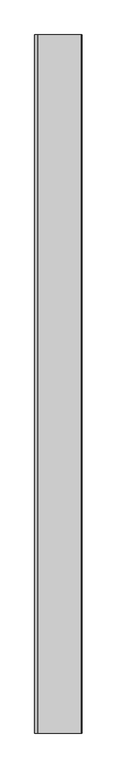
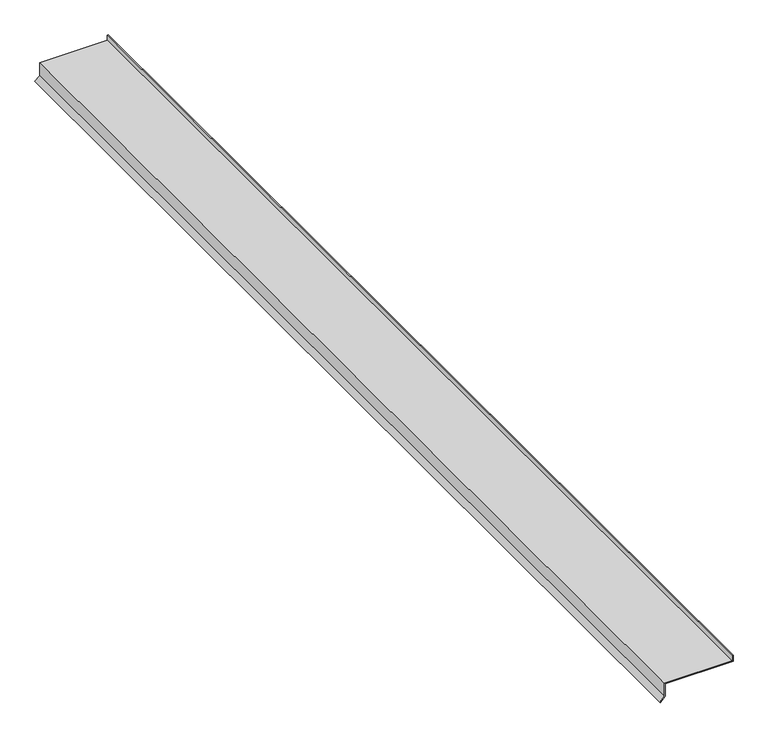
"""IFC4 building model written with IfcOpenShell, lengths in millimetres: proxy geometry, Flashing17:Flashing027:300321 : Flashing17:Flashing027:300321."""

from ifc_helpers import new_model, si_unit, frame, origin, place, context, project, spatial, polyline, outline, extrude, source, transform, mapped, element, save


def generic_models_79b0ea0f(model_context):
    return source(origin(), model_context, "Body", "SweptSolid", [
        extrude(outline(polyline([(40335.3398438, 3792.4641251), (40335.3398438, 3790.4641251), (40325.640625, 3790.4641251), (40325.640625, 3665.4319596), (40300.3872772, 3665.4319596), (40291.9157249, 3656.5536039), (40290.46875, 3657.9342789), (40299.53125, 3667.4319596), (40323.640625, 3667.4319596), (40323.640625, 3792.4641251), (40335.3398438, 3792.4641251)])), frame((0.0, -774.5581163, 0.0), z_axis=(0.0, 1.0, 0.0), x_axis=(0.0, 0.0, 1.0)), (0.0, 0.0, 1.0), 2000.0),
    ])


if __name__ == "__main__":
    model = new_model("IFC4")
    model_context = context("Model", 3, world=origin())
    ifc_project = project(units=[si_unit("LENGTHUNIT", "METRE", prefix="MILLI")], contexts=[model_context])
    site = spatial("IfcSite", under=ifc_project)
    building = spatial("IfcBuilding", under=site)
    placement = place(None, origin())
    generic_models_shape = generic_models_79b0ea0f(model_context)
    element("IfcBuildingElementProxy", 1, Name="Flashing17:Flashing027:300321 : Flashing17:Flashing027:300321", ObjectType="Flashing17:Flashing027:300321 : Flashing17:Flashing027:300321", at=placement, inside=building, context=model_context, shape_type="MappedRepresentation", body=[
        mapped(generic_models_shape, transform((0.0, 0.0, 0.0), x_axis=(1.0, 0.0, 0.0), y_axis=(0.0, 1.0, 0.0), z_axis=(0.0, 0.0, 1.0))),
    ])
    save(model, "model.ifc")

# Revit data of these elements
# Type "Flashing17:Flashing027:300321 : Flashing17:Flashing027:300321"
#   NameOverride = "Flashing17:Flashing027:300321"
#   ObjectTypeOverride = "Flashing17:Flashing027"
#   Reference = "Flashing027"
#   Category = "Generic Models"
#   Tag = "300321"
# Element 1 (IfcBuildingElementProxy, "Flashing17:Flashing027:300321 : Flashing17:Flashing027:300321")
#   Materials on its faces: "COPPER SILL PAN AT ALL EXTERIOR WINDOWS/DOORS PER DETAIL 1/A4.1"
# Materials
#   "COPPER SILL PAN AT ALL EXTERIOR WINDOWS/DOORS PER DETAIL 1/A4.1": class "Unassigned", colour RGB 255 170 255, transparency 0, Cost = 0
